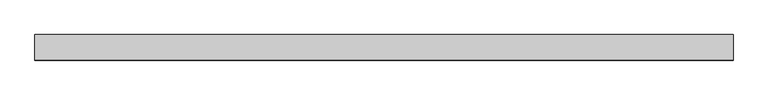
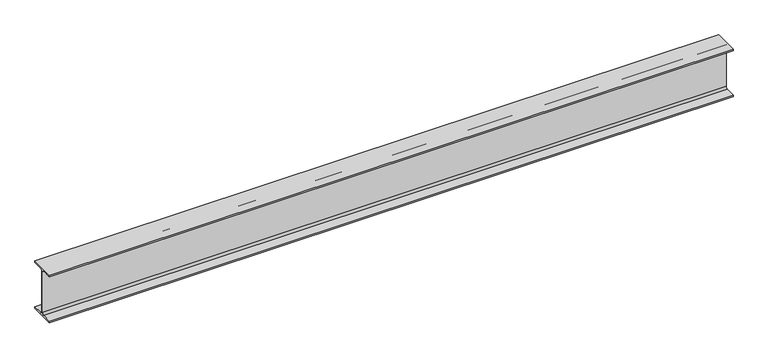
"""IFC4 building model written with IfcOpenShell, lengths in millimetres: beam geometry, 0912_Steel Framing_H-KSD3502 : H_SB_AR_S02_H-350x175x7x11_Platform."""

from ifc_helpers import new_model, si_unit, point, frame, frame_2d, origin, place, context, project, spatial, polyline, circle_curve, trimmed, segment, composite_curve, outline, extrude, source, transform, mapped, element, save


def beam_74d50635(model_context):
    return source(origin(), model_context, "Body", "SweptSolid", [
        extrude(outline(composite_curve([segment(polyline([(87.5, -164.0), (87.5, -175.0), (-87.5, -175.0), (-87.5, -164.0), (-17.5, -164.0)]), True, "CONTINUOUS"), segment(trimmed(circle_curve(frame_2d((-17.5, -150.0)), 14.0), [point((-17.5, -164.0))], [point((-3.5, -150.0))], True, "CARTESIAN"), True, "CONTINUOUS"), segment(polyline([(-3.5, -150.0), (-3.5, 150.0)]), True, "CONTINUOUS"), segment(trimmed(circle_curve(frame_2d((-17.5, 150.0)), 14.0), [point((-3.5, 150.0))], [point((-17.5, 164.0))], True, "CARTESIAN"), True, "CONTINUOUS"), segment(polyline([(-17.5, 164.0), (-87.5, 164.0), (-87.5, 175.0), (87.5, 175.0), (87.5, 164.0), (17.5, 164.0)]), True, "CONTINUOUS"), segment(trimmed(circle_curve(frame_2d((17.5, 150.0)), 14.0), [point((17.5, 164.0))], [point((3.5, 150.0))], True, "CARTESIAN"), True, "CONTINUOUS"), segment(polyline([(3.5, 150.0), (3.5, -150.0)]), True, "CONTINUOUS"), segment(trimmed(circle_curve(frame_2d((17.5, -150.0)), 14.0), [point((3.5, -150.0))], [point((17.5, -164.0))], True, "CARTESIAN"), True, "CONTINUOUS"), segment(polyline([(17.5, -164.0), (87.5, -164.0)]), True, "CONTINUOUS")], self_intersect=False)), frame((-2387.3, 0.0, 0.0), z_axis=(1.0, 0.0, 0.0), x_axis=(0.0, 1.0, 0.0)), (0.0, 0.0, 1.0), 4774.6),
    ])


if __name__ == "__main__":
    model = new_model("IFC4")
    model_context = context("Model", 3, world=origin())
    ifc_project = project(units=[si_unit("LENGTHUNIT", "METRE", prefix="MILLI")], contexts=[model_context])
    site = spatial("IfcSite", under=ifc_project)
    building = spatial("IfcBuilding", under=site)
    placement = place(None, origin())
    beam_shape = beam_74d50635(model_context)
    element("IfcBeam", 1, ObjectType="0912_Steel Framing_H-KSD3502 : H_SB_AR_S02_H-350x175x7x11_Platform", at=placement, inside=building, context=model_context, shape_type="MappedRepresentation", body=[
        mapped(beam_shape, transform((0.0, 0.0, 0.0), x_axis=(1.0, 0.0, 0.0), y_axis=(0.0, 1.0, 0.0), z_axis=(0.0, 0.0, 1.0))),
    ])
    save(model, "model.ifc")

# Revit data of these elements
# Type "0912_Steel Framing_H-KSD3502 : H_SB_AR_S02_H-350x175x7x11_Platform"
#   H_Q'ty Cal Type Tag = "SB-Q2"
#   H_WM Code_1 = "S01AA073-00001 |  | TON | Main Steel Structure Fabrication Work | Shelter/Building | Medium Steel - Standard |  |  |  |  |  |  | Material: (   ) | (90)KG/M>Weight≥(30)KG/M | S01AA073-00001 Main Steel Structure Fabrication Work Shelter/Building Medium Steel - Standard         | - Material: ( ASTM A36 )\n- (90)KG/M>Weight≥(30)KG/M"
#   H_WM Code_2 = "S03AA083-00001 |  | TON | Main Steel Structure Erection Work | Shelter/Building | Medium Steel |  |  |  |  |  |  | Material: (   ) | S03AA083-00001 Main Steel Structure Erection Work Shelter/Building Medium Steel         | - Material: ( ASTM A36 )"
#   H_WM Code_3 = "S01AA009-00001 |  | TON | Main Steel Structure Fabrication Work | Shelter/Building | Plates - Gusset, Stiffener, ETC | Material: (   ) | S01AA009-00001 Main Steel Structure Fabrication Work Shelter/Building Plates - Gusset, Stiffener, ETC         |"
#   H_WM Code_4 = "S41AA051-00001 |  | M2 | Steel Structure Paint Work | Shelter/Building | for Non-Fireproofed Steel Surface |  |  |  |  |  |  | Material: (   ) | S41AA051-00001 Steel Structure Paint Work Shelter/Building for Non-Fireproofed Steel Surface         |"
#   Width = 17.5 cm
#   Web Thickness = 0.7 cm
#   Web Fillet = 1.4 cm
#   Warping Constant = 282000.0 cm⁶
#   W = 0
#   Torsional Moment of Inertia = 19.4042 cm⁴
#   Section Area = 63.14 cm²
#   Plastic Modulus weak axis = 174.0 cm³
#   Plastic Modulus strong axis = 868.0 cm³
#   Perimeter = 1.36 m²/m
#   Nominal Weight = 49.60 kgf/m
#   Moment of Inertia weak axis = 984.00 cm⁴
#   Moment of Inertia strong axis = 13600.00 cm⁴
#   Height = 35.0 cm
#   Flange Thickness = 1.1 cm
#   Elastic Modulus weak axis = 112.0 cm³
#   Elastic Modulus strong axis = 775.0 cm³
#   Centroid Vertical = 17.5 cm
#   Centroid Horizontal = 8.75 cm
#   Ix = 136000000
#   Length [instance default] = 1524 mm
#   Zx = 868000
#   b = 175 mm
#   h = 350 mm
#   r = 14 mm
#   s = 7 mm
#   t = 11 mm
#   A = 0.006314 m²
#   Structural Material [instance default] = Steel, 45-345
#   Assembly Code = ""
# Element 1 (IfcBeam, "0912_Steel Framing_H-KSD3502 : H_SB_AR_S02_H-350x175x7x11_Platform")
#   Materials on its faces: "Steel, 45-345"
# Materials
#   "Steel, 45-345": class "Metal", colour RGB 189 187 185, transparency 0, Description = "Steel 345 MPa", Cost = 0
